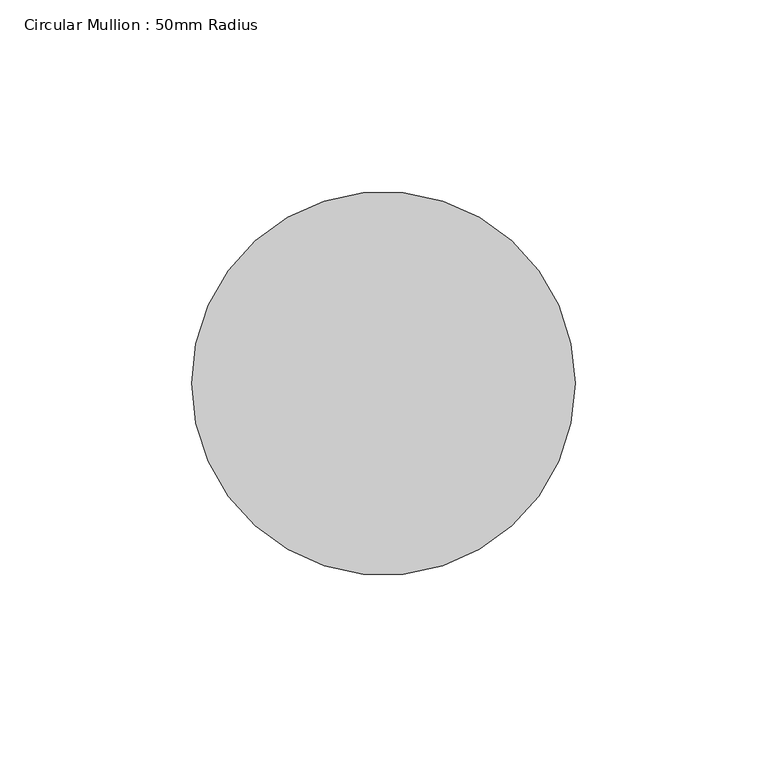
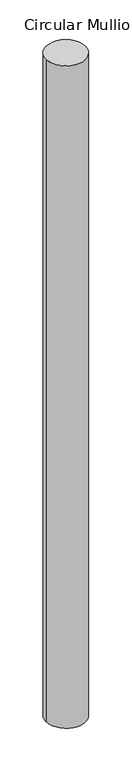
"""IFC4 building model written with IfcOpenShell, lengths in millimetres: member geometry, Circular Mullion : 50mm Radius."""

from ifc_helpers import new_model, si_unit, point, frame, origin, origin_2d, place, context, project, spatial, circle_curve, trimmed, segment, composite_curve, outline, extrude, source, transform, mapped, element, save


def circular_mullion_50mm_radius_5e04201a(model_context):
    return source(origin(), model_context, "Body", "SweptSolid", [
        extrude(outline(composite_curve([segment(trimmed(circle_curve(origin_2d(), 50.0), [point((50.0, 0.0))], [point((-50.0, 0.0))], False, "CARTESIAN"), True, "CONTINUOUS"), segment(trimmed(circle_curve(origin_2d(), 50.0), [point((-50.0, 0.0))], [point((50.0, 0.0))], False, "CARTESIAN"), True, "CONTINUOUS")], self_intersect=False)), frame((0.0, 0.0, -1768.5736381), z_axis=(0.0, 0.0, 1.0), x_axis=(1.0, 0.0, 0.0)), (0.0, 0.0, 1.0), 1768.5736381),
    ])


if __name__ == "__main__":
    model = new_model("IFC4")
    model_context = context("Model", 3, world=origin())
    ifc_project = project(units=[si_unit("LENGTHUNIT", "METRE", prefix="MILLI")], contexts=[model_context])
    site = spatial("IfcSite", under=ifc_project)
    building = spatial("IfcBuilding", under=site)
    placement = place(None, origin())
    circular_mullion_50mm_radius_shape = circular_mullion_50mm_radius_5e04201a(model_context)
    element("IfcMember", 1, ObjectType="Circular Mullion : 50mm Radius", at=placement, inside=building, context=model_context, shape_type="MappedRepresentation", body=[
        mapped(circular_mullion_50mm_radius_shape, transform((0.0, 0.0, 0.0), x_axis=(1.0, 0.0, 0.0), y_axis=(0.0, 1.0, 0.0), z_axis=(0.0, 0.0, 1.0))),
    ])
    save(model, "model.ifc")

# Revit data of these elements
# Type "Circular Mullion : 50mm Radius"
#   built-in parameter 1007350 = 0.164042 (stored number, unit not read)
# Element 1 (IfcMember, "Circular Mullion : 50mm Radius")
#   Materials on its faces: "Aluminium"
# Materials
#   "Aluminium": class "Metal", colour RGB 247 247 247, transparency 0, Description = "Aluminium 6061", Cost = 0
